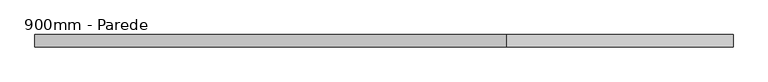
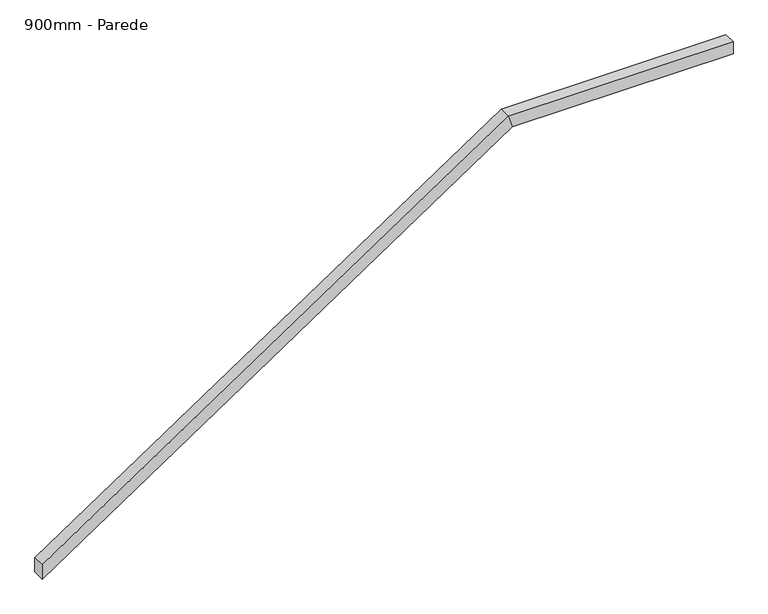
"""IFC4 building model written with IfcOpenShell, lengths in millimetres: railing geometry, 900mm - Parede."""

from ifc_helpers import new_model, si_unit, origin, place, context, project, spatial, faceted_brep, source, transform, mapped, element, save


def railing_900mm_parede_56b9a861(model_context):
    return source(origin(), model_context, "Body", "Brep", [
        faceted_brep([(-1574.4431325, -440.6624019, 1480.0), (-1574.4431325, -440.6624019, 1419.9074787), (-1574.4431325, -490.6624019, 1419.9074787), (-1574.4431325, -490.6624019, 1480.0), (315.5568675, -440.6624019, 2740.0), (330.6956494, -440.6624019, 2690.0), (330.6956494, -490.6624019, 2690.0), (315.5568675, -490.6624019, 2740.0), (1225.5568675, -440.6624019, 2740.0), (1225.5568675, -490.6624019, 2740.0), (1225.5568675, -490.6624019, 2690.0), (1225.5568675, -440.6624019, 2690.0)], [[[0, 1, 2, 3]], [[1, 0, 4, 5]], [[2, 1, 5, 6]], [[3, 2, 6, 7]], [[0, 3, 7, 4]], [[8, 9, 10, 11]], [[5, 4, 8, 11]], [[6, 5, 11, 10]], [[7, 6, 10, 9]], [[4, 7, 9, 8]]]),
    ])


if __name__ == "__main__":
    model = new_model("IFC4")
    model_context = context("Model", 3, world=origin())
    ifc_project = project(units=[si_unit("LENGTHUNIT", "METRE", prefix="MILLI")], contexts=[model_context])
    site = spatial("IfcSite", under=ifc_project)
    building = spatial("IfcBuilding", under=site)
    placement = place(None, origin())
    railing_900mm_parede_shape = railing_900mm_parede_56b9a861(model_context)
    element("IfcRailing", 1, ObjectType="900mm - Parede", at=placement, inside=building, context=model_context, shape_type="MappedRepresentation", body=[
        mapped(railing_900mm_parede_shape, transform((0.0, 0.0, 0.0), x_axis=(1.0, 0.0, 0.0), y_axis=(0.0, 1.0, 0.0), z_axis=(0.0, 0.0, 1.0))),
    ])
    save(model, "model.ifc")
